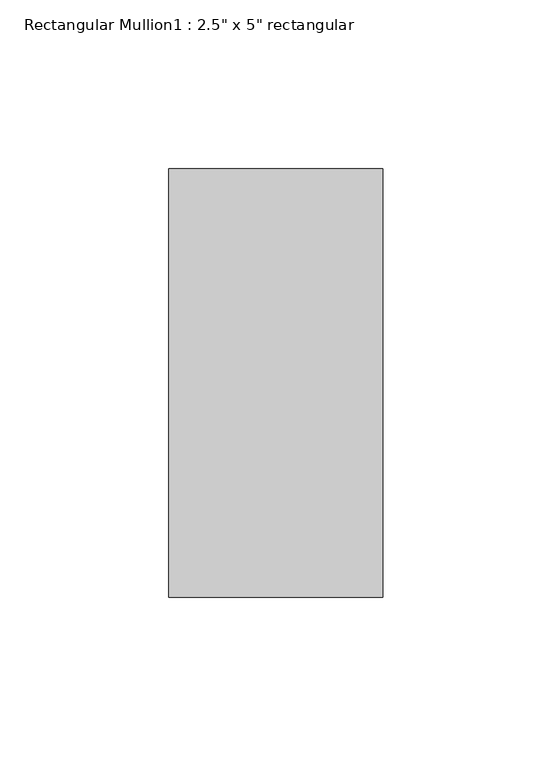
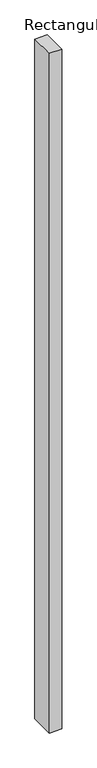
"""IFC4 building model written with IfcOpenShell, lengths in millimetres: member geometry."""

import ifcopenshell
import ifcopenshell.guid

model = None  # the IFC model being written
_history = None  # IfcOwnerHistory: only IFC2X3 demands one
_inside = {}  # id of a spatial element -> (the spatial element, [elements in it])
_under = {}  # id of a project, library or spatial element -> (it, [spatial elements below it])
_declared = {}  # id of a project -> (the project, [libraries it declares])
_typed = {}  # id of a type object -> (the type object, [elements of that type])
_made_of = {}  # id of a material, layer set ... -> (it, [elements and type objects made of it])


def new_model(schema):
    """Start an empty IFC model of exactly this schema.

    Asked for "IFC4X3", IfcOpenShell would pick the latest addendum, in which some entities
    have other attributes; the version numbers below select the first issue.
    IFC2X3 requires an IfcOwnerHistory on every rooted entity: one is made here for all.
    """
    global model, _history
    if schema == "IFC4X3":
        model = ifcopenshell.file(schema_version=(4, 3, 0, 0))
    else:
        model = ifcopenshell.file(schema=schema)
    _inside.clear()
    _under.clear()
    _declared.clear()
    _typed.clear()
    _made_of.clear()
    _history = None
    if model.schema == "IFC2X3":
        org = make("IfcOrganization", Name="unknown")
        user = make(
            "IfcPersonAndOrganization",
            ThePerson=make("IfcPerson", FamilyName="unknown"),
            TheOrganization=org,
        )
        app = make(
            "IfcApplication",
            ApplicationDeveloper=org,
            Version="unknown",
            ApplicationFullName="unknown",
            ApplicationIdentifier="unknown",
        )
        _history = make(
            "IfcOwnerHistory",
            OwningUser=user,
            OwningApplication=app,
            ChangeAction="ADDED",
            CreationDate=0,
        )
    return model


def make(cls, **values):
    """One entity of the class cls with the attributes given. An attribute that is None is left unset."""
    return model.create_entity(
        cls, **{name: value for name, value in values.items() if value is not None}
    )


def rooted(cls, **values):
    """An entity with a GlobalId (a new one), such as an element, a storey or a relation."""
    return make(cls, GlobalId=ifcopenshell.guid.new(), OwnerHistory=_history, **values)


def si_unit(unit_type, name, prefix=None):
    """IfcSIUnit, for example si_unit("LENGTHUNIT", "METRE", prefix="MILLI")."""
    return make("IfcSIUnit", UnitType=unit_type, Prefix=prefix, Name=name)


def assignment(units):
    """IfcUnitAssignment: the units of a project."""
    return None if units is None else make("IfcUnitAssignment", Units=units)


def point(xyz):
    """IfcCartesianPoint."""
    return None if xyz is None else make("IfcCartesianPoint", Coordinates=xyz)


def direction(xyz):
    """IfcDirection."""
    return None if xyz is None else make("IfcDirection", DirectionRatios=xyz)


def frame(location, z_axis=None, x_axis=None):
    """IfcAxis2Placement3D, a coordinate frame: its origin and axes. An axis left out is left unset."""
    return make(
        "IfcAxis2Placement3D",
        Location=point(location),
        Axis=direction(z_axis),
        RefDirection=direction(x_axis),
    )


def origin():
    """The frame at (0, 0, 0) with its axes left unset."""
    return frame((0.0, 0.0, 0.0))


def place(relative_to, where):
    """IfcLocalPlacement: puts the frame where relative to a parent placement (None: the world)."""
    return make(
        "IfcLocalPlacement", PlacementRelTo=relative_to, RelativePlacement=where
    )


def context(
    kind, dimensions, precision=None, world=None, true_north=None, identifier=None
):
    """IfcGeometricRepresentationContext, for example the 3D "Model" context."""
    return make(
        "IfcGeometricRepresentationContext",
        ContextIdentifier=identifier,
        ContextType=kind,
        CoordinateSpaceDimension=dimensions,
        Precision=precision,
        WorldCoordinateSystem=world,
        TrueNorth=true_north,
    )


def project(units=None, contexts=None):
    """IfcProject with its units and contexts."""
    return rooted(
        "IfcProject",
        Name="project",
        RepresentationContexts=contexts,
        UnitsInContext=assignment(units),
    )


def spatial(cls, under=None, at=None, **own):
    """A site, building, storey or space (cls), placed at a placement, below another one or the project."""
    s = rooted(cls, ObjectPlacement=at, **own)
    if under is not None:
        _under.setdefault(under.id(), (under, []))[1].append(s)
    return s


def polyline(points):
    """IfcPolyline through the points."""
    return make("IfcPolyline", Points=[point(p) for p in points])


def outline(outer, holes=None, kind="AREA"):
    """IfcArbitraryClosedProfileDef: a profile drawn as a closed curve; with holes, ...WithVoids."""
    if holes is None:
        return make("IfcArbitraryClosedProfileDef", ProfileType=kind, OuterCurve=outer)
    return make(
        "IfcArbitraryProfileDefWithVoids",
        ProfileType=kind,
        OuterCurve=outer,
        InnerCurves=holes,
    )


def extrude(swept, where, along, depth):
    """IfcExtrudedAreaSolid: the profile swept, set in the frame where, extruded along a direction by depth."""
    return make(
        "IfcExtrudedAreaSolid",
        SweptArea=swept,
        Position=where,
        ExtrudedDirection=direction(along),
        Depth=depth,
    )


def shape(context_of_items, identifier, shape_type, items):
    """IfcShapeRepresentation: the items that make up one representation, for example the "Body"."""
    return make(
        "IfcShapeRepresentation",
        ContextOfItems=context_of_items,
        RepresentationIdentifier=identifier,
        RepresentationType=shape_type,
        Items=items,
    )


def source(mapping_origin, context_of_items, identifier, shape_type, items):
    """IfcRepresentationMap: a shape defined once, which mapped items show again and again."""
    return make(
        "IfcRepresentationMap",
        MappingOrigin=mapping_origin,
        MappedRepresentation=shape(context_of_items, identifier, shape_type, items),
    )


def transform(
    local_origin,
    x_axis=None,
    y_axis=None,
    z_axis=None,
    scale=None,
    scale2=None,
    scale3=None,
    uniform=True,
):
    """IfcCartesianTransformationOperator3D, or its non-uniform kind. x_axis, y_axis, z_axis: its Axis1, 2, 3."""
    if uniform:
        return make(
            "IfcCartesianTransformationOperator3D",
            Axis1=direction(x_axis),
            Axis2=direction(y_axis),
            LocalOrigin=point(local_origin),
            Scale=scale,
            Axis3=direction(z_axis),
        )
    return make(
        "IfcCartesianTransformationOperator3DnonUniform",
        Axis1=direction(x_axis),
        Axis2=direction(y_axis),
        LocalOrigin=point(local_origin),
        Scale=scale,
        Axis3=direction(z_axis),
        Scale2=scale2,
        Scale3=scale3,
    )


def mapped(mapping_source, mapping_target):
    """IfcMappedItem: shows the shape of a source again, moved by a transform."""
    return make(
        "IfcMappedItem", MappingSource=mapping_source, MappingTarget=mapping_target
    )


def made_of(thing, what):
    """Note that an element or type object is made of a material, layer set ...; save() writes the relation."""
    if what is not None:
        _made_of.setdefault(what.id(), (what, []))[1].append(thing)
    return thing


def element(
    cls,
    number,
    at=None,
    inside=None,
    cuts=None,
    type_object=None,
    material=None,
    context=None,
    identifier="Body",
    shape_type=None,
    held_by="IfcProductDefinitionShape",
    body=None,
    shapes=None,
    **own,
):
    """One element of the class cls, such as IfcWall. Its Tag is "e" and its number.

    at: its placement. inside: the storey or other place that contains it. cuts: it is an
    opening in that element (IfcRelVoidsElement). A single representation is given by context,
    identifier, shape_type and body (its items); several are given by shapes. held_by: the class
    of the entity that holds the representations. save() writes the other relations.
    """
    e = rooted(cls, Tag="e%d" % number, ObjectPlacement=at, **own)
    if body is not None:
        shapes = [shape(context, identifier, shape_type, body)]
    if shapes is not None:
        e.Representation = make(held_by, Representations=shapes)
    if inside is not None:
        _inside.setdefault(inside.id(), (inside, []))[1].append(e)
    if cuts is not None:
        rooted(
            "IfcRelVoidsElement", RelatingBuildingElement=cuts, RelatedOpeningElement=e
        )
    if type_object is not None:
        _typed.setdefault(type_object.id(), (type_object, []))[1].append(e)
    return made_of(e, material)


def aggregate(whole, parts):
    """IfcRelAggregates: a whole, such as a stair, and the parts it consists of."""
    return rooted("IfcRelAggregates", RelatingObject=whole, RelatedObjects=parts)


def save(model, path):
    """Write the relations noted so far, then the file.

    IfcRelAggregates (storeys below a building ...), IfcRelContainedInSpatialStructure (elements
    in a storey), IfcRelDefinesByType, IfcRelAssociatesMaterial and IfcRelDeclares: one each for
    every whole, place, type object, material and project.
    """
    for whole, parts in _under.values():
        aggregate(whole, parts)
    for where, things in _inside.values():
        rooted(
            "IfcRelContainedInSpatialStructure",
            RelatedElements=things,
            RelatingStructure=where,
        )
    for kind, things in _typed.values():
        rooted("IfcRelDefinesByType", RelatedObjects=things, RelatingType=kind)
    for what, things in _made_of.values():
        rooted("IfcRelAssociatesMaterial", RelatedObjects=things, RelatingMaterial=what)
    for by, libraries in _declared.values():
        rooted("IfcRelDeclares", RelatingContext=by, RelatedDefinitions=libraries)
    model.write(path)


def member_810865a4(model_context):
    return source(origin(), model_context, "Body", "SweptSolid", [
        extrude(outline(polyline([(31.75, 63.5), (31.75, -63.5), (-31.75, -63.5), (-31.75, 63.5), (31.75, 63.5)])), frame((0.0, 0.0, -3657.6), z_axis=(0.0, 0.0, 1.0), x_axis=(1.0, 0.0, 0.0)), (0.0, 0.0, 1.0), 3657.6),
    ])


if __name__ == "__main__":
    model = new_model("IFC4")
    model_context = context("Model", 3, world=origin())
    ifc_project = project(units=[si_unit("LENGTHUNIT", "METRE", prefix="MILLI")], contexts=[model_context])
    site = spatial("IfcSite", under=ifc_project)
    building = spatial("IfcBuilding", under=site)
    placement = place(None, origin())
    member_shape = member_810865a4(model_context)
    element("IfcMember", 1, ObjectType="Rectangular Mullion1 : 2.5\" x 5\" rectangular", at=placement, inside=building, context=model_context, shape_type="MappedRepresentation", body=[
        mapped(member_shape, transform((0.0, 0.0, 0.0), x_axis=(1.0, 0.0, 0.0), y_axis=(0.0, 1.0, 0.0), z_axis=(0.0, 0.0, 1.0))),
    ])
    save(model, "model.ifc")

# Revit data of these elements
# Type "Rectangular Mullion1 : 2.5\" x 5\" rectangular"
#   built-in parameter 1007304 = 0.416667 (stored number, unit not read)
#   built-in parameter 1007301 = 0.104167 (stored number, unit not read)
#   built-in parameter 1007300 = 0.104167 (stored number, unit not read)
# Element 1 (IfcMember, "Rectangular Mullion1 : 2.5\" x 5\" rectangular")
#   Materials on its faces: "support-frame"
# Materials
#   "support-frame": class "Unassigned", colour RGB 233 233 233, transparency 0, Cost = 0
